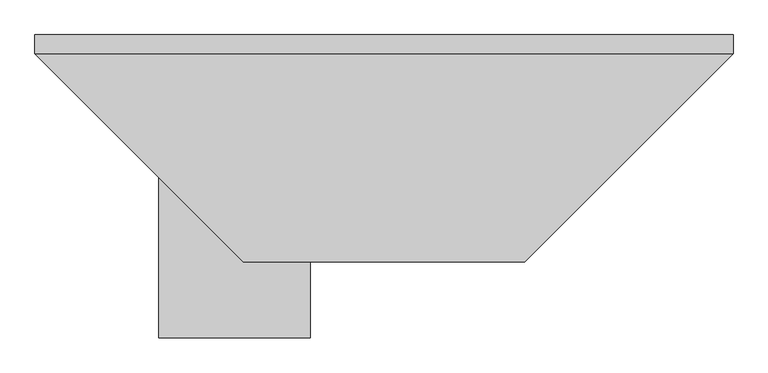
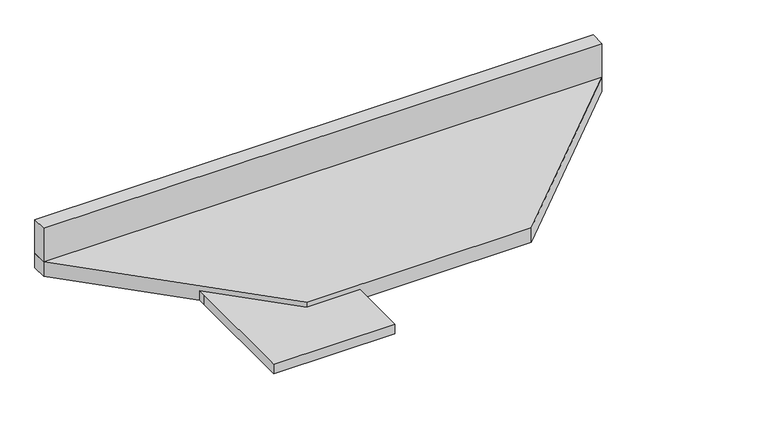
"""IFC4 building model written with IfcOpenShell, lengths in millimetres: proxy geometry, CT020 - Countertop, SS, No Opening - Angled-1 : CT020 - Countertop, SS, No Opening - Angled-1."""

from ifc_helpers import new_model, si_unit, frame, origin, place, context, project, spatial, polyline, outline, extrude, source, transform, mapped, element, save


def specialty_equipment_c0fcd640(model_context):
    return source(origin(), model_context, "Body", "SweptSolid", [
        extrude(outline(polyline([(-400.9054372, 266.7), (-400.9054372, 304.8), (1002.6430003, 304.8), (1002.6430003, 266.7), (-400.9054372, 266.7)])), frame((0.0, 0.0, 876.3), z_axis=(0.0, 0.0, 1.0), x_axis=(1.0, 0.0, 0.0)), (0.0, 0.0, 1.0), 88.9),
        extrude(outline(polyline([(1002.6430003, 304.8), (1002.6430003, 266.6686289), (583.5743714, -152.4), (18.2130614, -152.4), (-400.9054372, 266.7184987), (-400.9054372, 304.8), (1002.6430003, 304.8)])), frame((0.0, 0.0, 838.2), z_axis=(0.0, 0.0, 1.0), x_axis=(1.0, 0.0, 0.0)), (0.0, 0.0, 1.0), 38.1),
        extrude(outline(polyline([(-152.4, 304.8), (152.4, 304.8), (152.4, -304.8), (-152.4, -304.8), (-152.4, 0.0), (-152.4, 304.8)])), frame((0.0, 0.0, 838.2), z_axis=(0.0, 0.0, 1.0), x_axis=(1.0, 0.0, 0.0)), (0.0, 0.0, 1.0), 25.4),
    ])


if __name__ == "__main__":
    model = new_model("IFC4")
    model_context = context("Model", 3, world=origin())
    ifc_project = project(units=[si_unit("LENGTHUNIT", "METRE", prefix="MILLI")], contexts=[model_context])
    site = spatial("IfcSite", under=ifc_project)
    building = spatial("IfcBuilding", under=site)
    placement = place(None, origin())
    specialty_equipment_shape = specialty_equipment_c0fcd640(model_context)
    element("IfcBuildingElementProxy", 1, Name="CT020 - Countertop, SS, No Opening - Angled-1 : CT020 - Countertop, SS, No Opening - Angled-1", ObjectType="CT020 - Countertop, SS, No Opening - Angled-1 : CT020 - Countertop, SS, No Opening - Angled-1", at=placement, inside=building, context=model_context, shape_type="MappedRepresentation", body=[
        mapped(specialty_equipment_shape, transform((0.0, 0.0, 0.0), x_axis=(1.0, 0.0, 0.0), y_axis=(0.0, 1.0, 0.0), z_axis=(0.0, 0.0, 1.0))),
    ])
    save(model, "model.ifc")

# Revit data of these elements
# Project information
#   Sheets - Total = "5"
#   Project Issue Date = "Issue Date"
#   Project Status = "Project Status"
#   Client Name = "Owner"
#   Project Address = "Enter address here"
#   Project Name = "Project Name"
#   Project Number = "Project Number"
#   Publication Date = "30-Jan-15"
# Type "CT020 - Countertop, SS, No Opening - Angled-1 : CT020 - Countertop, SS, No Opening - Angled-1"
#   Watts2 = "0"
#   Watts1 = "0"
#   Unit_Issue = "LF"
#   UTIL_6_Misc = "-"
#   UTIL_5_NonMedGas = "-"
#   UTIL_4_MiscGas = "-"
#   UTIL_3_MedGas = "-"
#   UTIL_2_Elec = "-"
#   UTIL_1_WaterDrain = "-"
#   Nomenclature = "Countertop, Solid Surface, Angled"
#   NSN = ""
#   Location [instance default] = ""
#   JSN = "CT020"
#   Fund_Source_VA = "-"
#   Fund_Source_Navy = "-"
#   Fund_Source_Army = "-"
#   Fund_Source_AF = "-"
#   ELEC_Volts2 = "0"
#   ELEC_Volts1 = "0"
#   ELEC_Phase2 = "0"
#   ELEC_Phase1 = "0"
#   ELEC_HertzSwitch = "0"
#   ELEC_HertzDependent = "0"
#   ELEC_Hertz = "0"
#   ELEC_Amps2 = "0"
#   ELEC_Amps1 = "0"
#   DetailDescription = ""
#   CAT_VA = "A"
#   CAT_Navy = "A"
#   CAT_IHS = "-"
#   CAT_Army = "A"
#   CAT_AF = "A"
#   BTUperhour = "0"
#   Weight_IP = 14
#   DIM_Width_IP = 1' - 0"
#   DIM_Height_IP = 0' - 1"
#   DIM_Depth_IP = 2' - 0"
#   CustomLength [instance default] = 4' - 0"
#   Assembly Code = ""
# Element 1 (IfcBuildingElementProxy, "CT020 - Countertop, SS, No Opening - Angled-1 : CT020 - Countertop, SS, No Opening - Angled-1")
#   Materials on its faces: "CounterTopFinish", "EquipSpace"
# Materials
#   "CounterTopFinish": class "Unassigned", colour RGB 139 121 96, transparency 0
#   "EquipSpace": class "Unassigned", colour RGB 221 217 195, transparency 0.5
